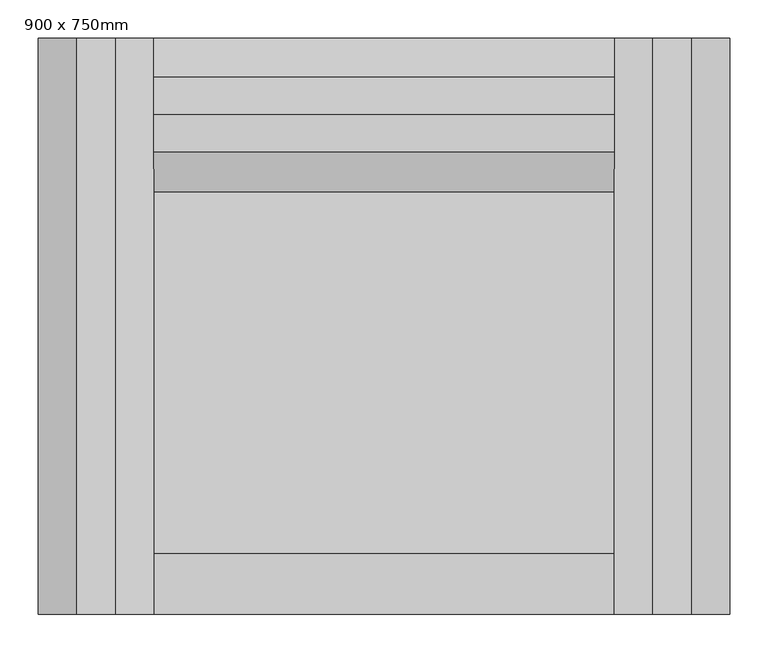
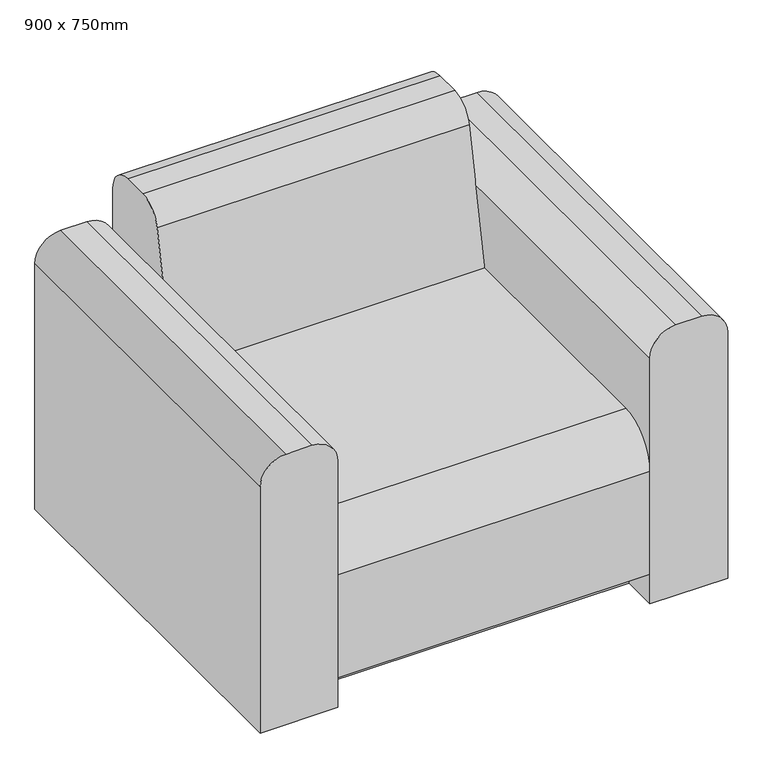
"""IFC4 building model written with IfcOpenShell, lengths in millimetres: furniture geometry, ソファ－I型 : 900 x 750mm."""

from ifc_helpers import new_model, si_unit, point, frame, frame_2d, origin, place, context, project, spatial, polyline, circle_curve, trimmed, segment, composite_curve, outline, extrude, source, transform, mapped, element, save


def furniture_900_x_750mm_ff71e519(model_context):
    return source(origin(), model_context, "Body", "SweptSolid", [
        extrude(outline(composite_curve([segment(trimmed(circle_curve(frame_2d((500.0, -400.0)), 50.0), [point((550.0, -400.0))], [point((500.0, -450.0))], False, "CARTESIAN"), True, "CONTINUOUS"), segment(polyline([(500.0, -450.0), (0.0, -450.0), (0.0, -300.0), (500.0, -300.0)]), True, "CONTINUOUS"), segment(trimmed(circle_curve(frame_2d((500.0, -350.0)), 50.0), [point((500.0, -300.0))], [point((550.0, -350.0))], False, "CARTESIAN"), True, "CONTINUOUS"), segment(polyline([(550.0, -350.0), (550.0, -400.0)]), True, "CONTINUOUS")], self_intersect=False)), frame((0.0, -375.0, 0.0), z_axis=(0.0, 1.0, 0.0), x_axis=(0.0, 0.0, 1.0)), (0.0, 0.0, 1.0), 750.0),
        extrude(outline(composite_curve([segment(polyline([(550.0, 400.0), (550.0, 350.0)]), True, "CONTINUOUS"), segment(trimmed(circle_curve(frame_2d((500.0, 350.0)), 50.0), [point((550.0, 350.0))], [point((500.0, 300.0))], False, "CARTESIAN"), True, "CONTINUOUS"), segment(polyline([(500.0, 300.0), (0.0, 300.0), (0.0, 450.0), (500.0, 450.0)]), True, "CONTINUOUS"), segment(trimmed(circle_curve(frame_2d((500.0, 400.0)), 50.0), [point((500.0, 450.0))], [point((550.0, 400.0))], False, "CARTESIAN"), True, "CONTINUOUS")], self_intersect=False)), frame((0.0, -375.0, 0.0), z_axis=(0.0, 1.0, 0.0), x_axis=(0.0, 0.0, 1.0)), (0.0, 0.0, 1.0), 750.0),
        extrude(outline(composite_curve([segment(trimmed(circle_curve(frame_2d((275.9901951, 600.0)), 50.0), [point((226.9611614, 609.8058068))], [point((275.9901951, 650.0))], False, "CARTESIAN"), True, "CONTINUOUS"), segment(polyline([(275.9901951, 650.0), (325.0, 650.0)]), True, "CONTINUOUS"), segment(trimmed(circle_curve(frame_2d((325.0, 600.0)), 50.0), [point((325.0, 650.0))], [point((375.0, 600.0))], False, "CARTESIAN"), True, "CONTINUOUS"), segment(polyline([(375.0, 600.0), (375.0, 0.0), (-305.0, 0.0), (-305.0, 60.0), (-375.0, 60.0), (-375.0, 270.0)]), True, "CONTINUOUS"), segment(trimmed(circle_curve(frame_2d((-295.0, 270.0)), 80.0), [point((-375.0, 270.0))], [point((-295.0, 350.0))], False, "CARTESIAN"), True, "CONTINUOUS"), segment(polyline([(-295.0, 350.0), (175.0, 350.0), (226.9611614, 609.8058068)]), True, "CONTINUOUS")], self_intersect=False)), frame((-300.0, 0.0, 0.0), z_axis=(1.0, 0.0, 0.0), x_axis=(0.0, 1.0, 0.0)), (0.0, 0.0, 1.0), 600.0),
    ])


if __name__ == "__main__":
    model = new_model("IFC4")
    model_context = context("Model", 3, world=origin())
    ifc_project = project(units=[si_unit("LENGTHUNIT", "METRE", prefix="MILLI")], contexts=[model_context])
    site = spatial("IfcSite", under=ifc_project)
    building = spatial("IfcBuilding", under=site)
    placement = place(None, origin())
    furniture_900_x_750mm_shape = furniture_900_x_750mm_ff71e519(model_context)
    element("IfcFurniture", 1, ObjectType="ソファ－I型 : 900 x 750mm", at=placement, inside=building, context=model_context, shape_type="MappedRepresentation", body=[
        mapped(furniture_900_x_750mm_shape, transform((0.0, 0.0, 0.0), x_axis=(1.0, 0.0, 0.0), y_axis=(0.0, 1.0, 0.0), z_axis=(0.0, 0.0, 1.0))),
    ])
    save(model, "model.ifc")

# Revit data of these elements
# Type "ソファ－I型 : 900 x 750mm"
#   Keynote = "12490.Y1"
#   座面高さ = 350 mm
#   幅 = 900 mm
#   奥行き = 750 mm
#   本体 = モチアミ - 無地 - グレー
#   Default Elevation = 0
# Element 1 (IfcFurniture, "ソファ－I型 : 900 x 750mm")
#   Materials on its faces: "モチアミ - 無地 - グレー"
# Materials
#   "モチアミ - 無地 - グレー": class "モチアミ", colour RGB 65 63 65, transparency 0, Cost = 0
